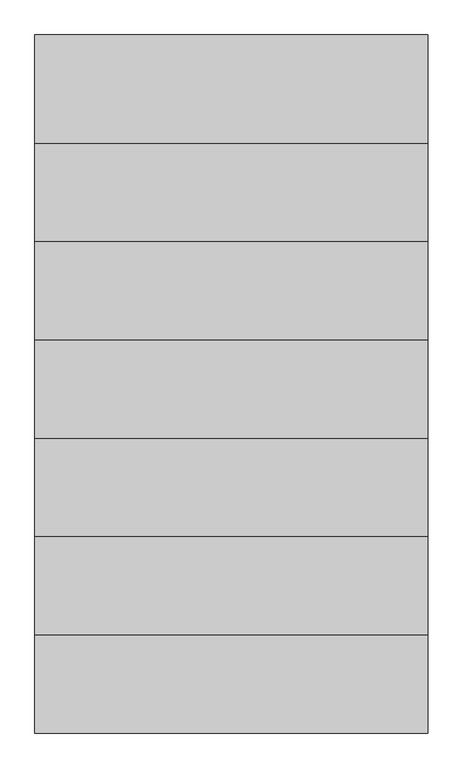
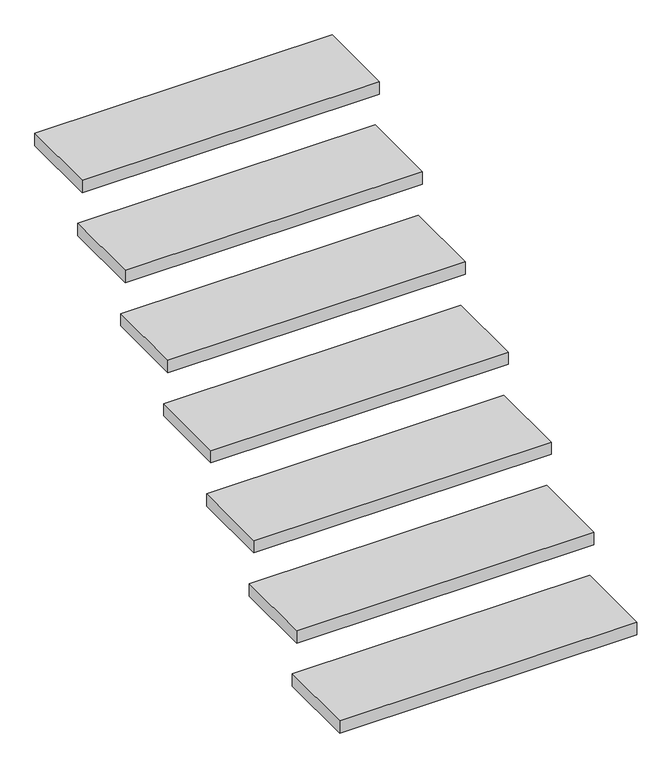
"""IFC4 building model written with IfcOpenShell, lengths in millimetres: stair flight geometry."""

from ifc_helpers import new_model, si_unit, frame, origin, place, context, project, spatial, polyline, outline, extrude, source, transform, mapped, element, save


def stair_flight_9550d146(model_context):
    return source(origin(), model_context, "Body", "SweptSolid", [
        extrude(outline(polyline([(-56846.2723171, 248819.549125), (-55830.2723171, 248819.549125), (-55830.2723171, 248540.149125), (-56846.2723171, 248540.149125), (-56846.2723171, 248819.549125)])), frame((0.0, 0.0, 1498.6), z_axis=(0.0, 0.0, 1.0), x_axis=(1.0, 0.0, 0.0)), (0.0, 0.0, 1.0), 44.45),
        extrude(outline(polyline([(-56846.2723171, 249073.549125), (-55830.2723171, 249073.549125), (-55830.2723171, 248794.149125), (-56846.2723171, 248794.149125), (-56846.2723171, 249073.549125)])), frame((0.0, 0.0, 1670.05), z_axis=(0.0, 0.0, 1.0), x_axis=(1.0, 0.0, 0.0)), (0.0, 0.0, 1.0), 44.45),
        extrude(outline(polyline([(-56846.2723171, 249327.549125), (-55830.2723171, 249327.549125), (-55830.2723171, 249048.149125), (-56846.2723171, 249048.149125), (-56846.2723171, 249327.549125)])), frame((0.0, 0.0, 1841.5), z_axis=(0.0, 0.0, 1.0), x_axis=(1.0, 0.0, 0.0)), (0.0, 0.0, 1.0), 44.45),
        extrude(outline(polyline([(-56846.2723171, 249581.549125), (-55830.2723171, 249581.549125), (-55830.2723171, 249302.149125), (-56846.2723171, 249302.149125), (-56846.2723171, 249581.549125)])), frame((0.0, 0.0, 2012.95), z_axis=(0.0, 0.0, 1.0), x_axis=(1.0, 0.0, 0.0)), (0.0, 0.0, 1.0), 44.45),
        extrude(outline(polyline([(-56846.2723171, 249835.549125), (-55830.2723171, 249835.549125), (-55830.2723171, 249556.149125), (-56846.2723171, 249556.149125), (-56846.2723171, 249835.549125)])), frame((0.0, 0.0, 2184.4), z_axis=(0.0, 0.0, 1.0), x_axis=(1.0, 0.0, 0.0)), (0.0, 0.0, 1.0), 44.45),
        extrude(outline(polyline([(-56846.2723171, 250089.549125), (-55830.2723171, 250089.549125), (-55830.2723171, 249810.149125), (-56846.2723171, 249810.149125), (-56846.2723171, 250089.549125)])), frame((0.0, 0.0, 2355.85), z_axis=(0.0, 0.0, 1.0), x_axis=(1.0, 0.0, 0.0)), (0.0, 0.0, 1.0), 44.45),
        extrude(outline(polyline([(-56846.2723171, 250343.549125), (-55830.2723171, 250343.549125), (-55830.2723171, 250064.149125), (-56846.2723171, 250064.149125), (-56846.2723171, 250343.549125)])), frame((0.0, 0.0, 2527.3), z_axis=(0.0, 0.0, 1.0), x_axis=(1.0, 0.0, 0.0)), (0.0, 0.0, 1.0), 44.45),
    ])


if __name__ == "__main__":
    model = new_model("IFC4")
    model_context = context("Model", 3, world=origin())
    ifc_project = project(units=[si_unit("LENGTHUNIT", "METRE", prefix="MILLI")], contexts=[model_context])
    site = spatial("IfcSite", under=ifc_project)
    building = spatial("IfcBuilding", under=site)
    placement = place(None, origin())
    stair_flight_shape = stair_flight_9550d146(model_context)
    element("IfcStairFlight", 1, at=placement, inside=building, context=model_context, shape_type="MappedRepresentation", body=[
        mapped(stair_flight_shape, transform((0.0, 0.0, 0.0), x_axis=(1.0, 0.0, 0.0), y_axis=(0.0, 1.0, 0.0), z_axis=(0.0, 0.0, 1.0))),
    ])
    save(model, "model.ifc")

# Revit data of these elements
# Element 1 (IfcStairFlight)
#   Materials on its faces: "Wood - Flooring"
# Materials
#   "Wood - Flooring": class "Unassigned", colour RGB 216 169 114, transparency 0
